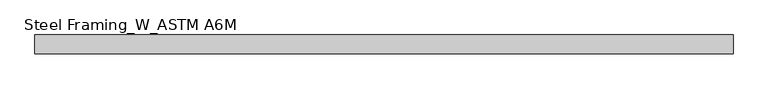
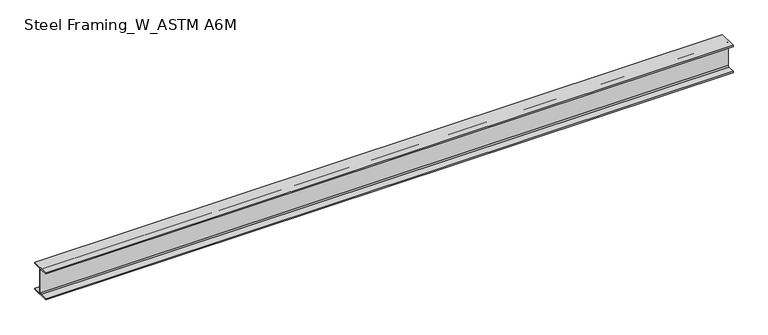
"""IFC4 building model written with IfcOpenShell, lengths in millimetres: beam geometry, Steel Framing_W_ASTM A6M : H_SB_AR_S02_W200x31.3_RB4."""

from ifc_helpers import new_model, si_unit, point, frame, frame_2d, origin, place, context, project, spatial, polyline, circle_curve, trimmed, segment, composite_curve, outline, extrude, source, transform, mapped, element, save


def steel_framing_w_astm_a6m_565b4d53(model_context):
    return source(origin(), model_context, "Body", "SweptSolid", [
        extrude(outline(composite_curve([segment(polyline([(67.0, -94.8), (67.0, -105.0), (-67.0, -105.0), (-67.0, -94.8), (-10.775, -94.8)]), True, "CONTINUOUS"), segment(trimmed(circle_curve(frame_2d((-10.775, -87.2)), 7.6), [point((-10.775, -94.8))], [point((-3.175, -87.2))], True, "CARTESIAN"), True, "CONTINUOUS"), segment(polyline([(-3.175, -87.2), (-3.175, 87.2)]), True, "CONTINUOUS"), segment(trimmed(circle_curve(frame_2d((-10.775, 87.2)), 7.6), [point((-3.175, 87.2))], [point((-10.775, 94.8))], True, "CARTESIAN"), True, "CONTINUOUS"), segment(polyline([(-10.775, 94.8), (-67.0, 94.8), (-67.0, 105.0), (67.0, 105.0), (67.0, 94.8), (10.775, 94.8)]), True, "CONTINUOUS"), segment(trimmed(circle_curve(frame_2d((10.775, 87.2)), 7.6), [point((10.775, 94.8))], [point((3.175, 87.2))], True, "CARTESIAN"), True, "CONTINUOUS"), segment(polyline([(3.175, 87.2), (3.175, -87.2)]), True, "CONTINUOUS"), segment(trimmed(circle_curve(frame_2d((10.775, -87.2)), 7.6), [point((3.175, -87.2))], [point((10.775, -94.8))], True, "CARTESIAN"), True, "CONTINUOUS"), segment(polyline([(10.775, -94.8), (67.0, -94.8)]), True, "CONTINUOUS")], self_intersect=False)), frame((-2500.0, 0.0, 0.0), z_axis=(1.0, 0.0, 0.0), x_axis=(0.0, 1.0, 0.0)), (0.0, 0.0, 1.0), 5000.0),
    ])


if __name__ == "__main__":
    model = new_model("IFC4")
    model_context = context("Model", 3, world=origin())
    ifc_project = project(units=[si_unit("LENGTHUNIT", "METRE", prefix="MILLI")], contexts=[model_context])
    site = spatial("IfcSite", under=ifc_project)
    building = spatial("IfcBuilding", under=site)
    placement = place(None, origin())
    steel_framing_w_astm_a6m_shape = steel_framing_w_astm_a6m_565b4d53(model_context)
    element("IfcBeam", 1, ObjectType="Steel Framing_W_ASTM A6M : H_SB_AR_S02_W200x31.3_RB4", at=placement, inside=building, context=model_context, shape_type="MappedRepresentation", body=[
        mapped(steel_framing_w_astm_a6m_shape, transform((0.0, 0.0, 0.0), x_axis=(1.0, 0.0, 0.0), y_axis=(0.0, 1.0, 0.0), z_axis=(0.0, 0.0, 1.0))),
    ])
    save(model, "model.ifc")

# Revit data of these elements
# Type "Steel Framing_W_ASTM A6M : H_SB_AR_S02_W200x31.3_RB4"
#   Type Mark = "RB4"
#   Section Name Key = "W8x21"
#   Width = 13.4 cm
#   Web Thickness = 0.635 cm
#   Web Fillet = 0.76 cm
#   Warping Constant = 40800.0 cm⁶
#   Torsional Moment of Inertia = 11.70 cm⁴
#   Section Area = 39.7 cm²
#   Plastic Modulus weak axis = 93.2 cm³
#   Plastic Modulus strong axis = 334.0 cm³
#   Perimeter = 0.93 m²/m
#   Nominal Weight = 31.30 kgf/m
#   Moment of Inertia weak axis = 407.00 cm⁴
#   Moment of Inertia strong axis = 3130.00 cm⁴
#   Height = 21.0 cm
#   Flange Thickness = 1.02 cm
#   Elastic Modulus weak axis = 60.8 cm³
#   Elastic Modulus strong axis = 298.0 cm³
#   Centroid Vertical = 10.5 cm
#   Centroid Horizontal = 6.7 cm
#   Length [instance default] = 1500 mm
#   Structural Material [instance default] = Steel, 45-345
#   Bolt Spacing = 0
#   Assembly Code = ""
# Element 1 (IfcBeam, "Steel Framing_W_ASTM A6M : H_SB_AR_S02_W200x31.3_RB4")
#   Materials on its faces: "Steel, 45-345"
# Materials
#   "Steel, 45-345": class "Metal", colour RGB 189 187 185, transparency 0, Description = "Steel 345 MPa", Cost = 0
